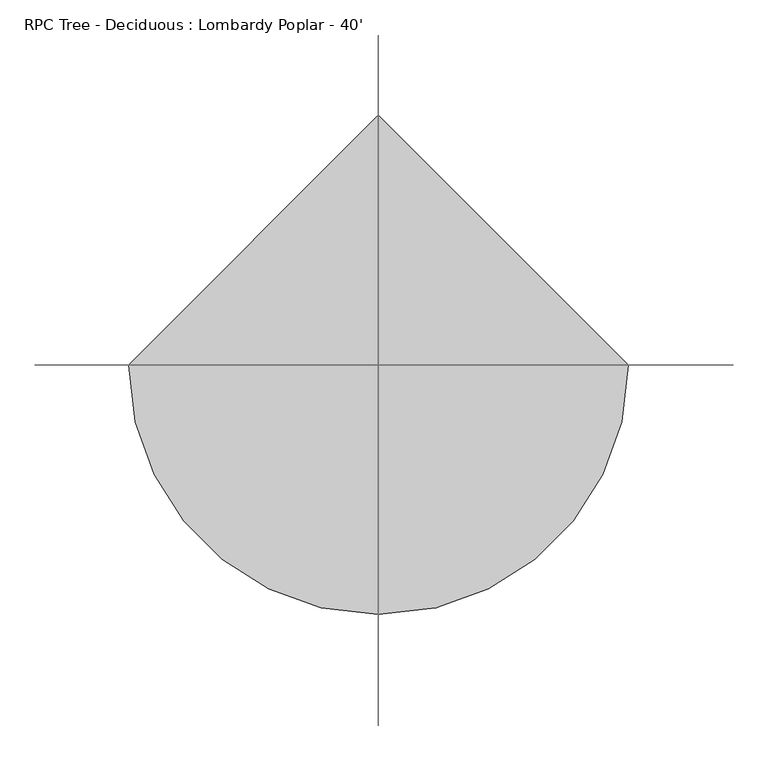
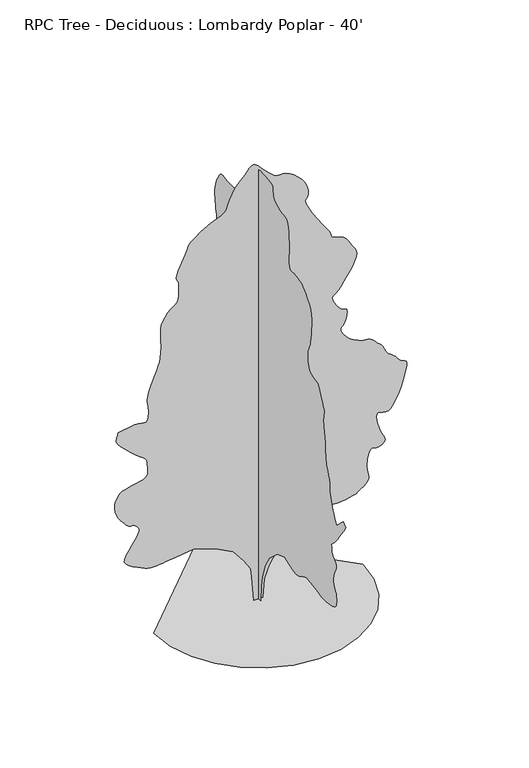
"""IFC4 building model written with IfcOpenShell, lengths in millimetres: geographic element geometry, RPC Tree - Deciduous : Lombardy Poplar - 40'."""

import ifcopenshell
import ifcopenshell.guid

model = None  # the IFC model being written
_history = None  # IfcOwnerHistory: only IFC2X3 demands one
_inside = {}  # id of a spatial element -> (the spatial element, [elements in it])
_under = {}  # id of a project, library or spatial element -> (it, [spatial elements below it])
_declared = {}  # id of a project -> (the project, [libraries it declares])
_typed = {}  # id of a type object -> (the type object, [elements of that type])
_made_of = {}  # id of a material, layer set ... -> (it, [elements and type objects made of it])


def new_model(schema):
    """Start an empty IFC model of exactly this schema.

    Asked for "IFC4X3", IfcOpenShell would pick the latest addendum, in which some entities
    have other attributes; the version numbers below select the first issue.
    IFC2X3 requires an IfcOwnerHistory on every rooted entity: one is made here for all.
    """
    global model, _history
    if schema == "IFC4X3":
        model = ifcopenshell.file(schema_version=(4, 3, 0, 0))
    else:
        model = ifcopenshell.file(schema=schema)
    _inside.clear()
    _under.clear()
    _declared.clear()
    _typed.clear()
    _made_of.clear()
    _history = None
    if model.schema == "IFC2X3":
        org = make("IfcOrganization", Name="unknown")
        user = make(
            "IfcPersonAndOrganization",
            ThePerson=make("IfcPerson", FamilyName="unknown"),
            TheOrganization=org,
        )
        app = make(
            "IfcApplication",
            ApplicationDeveloper=org,
            Version="unknown",
            ApplicationFullName="unknown",
            ApplicationIdentifier="unknown",
        )
        _history = make(
            "IfcOwnerHistory",
            OwningUser=user,
            OwningApplication=app,
            ChangeAction="ADDED",
            CreationDate=0,
        )
    return model


def make(cls, **values):
    """One entity of the class cls with the attributes given. An attribute that is None is left unset."""
    return model.create_entity(
        cls, **{name: value for name, value in values.items() if value is not None}
    )


def rooted(cls, **values):
    """An entity with a GlobalId (a new one), such as an element, a storey or a relation."""
    return make(cls, GlobalId=ifcopenshell.guid.new(), OwnerHistory=_history, **values)


def si_unit(unit_type, name, prefix=None):
    """IfcSIUnit, for example si_unit("LENGTHUNIT", "METRE", prefix="MILLI")."""
    return make("IfcSIUnit", UnitType=unit_type, Prefix=prefix, Name=name)


def assignment(units):
    """IfcUnitAssignment: the units of a project."""
    return None if units is None else make("IfcUnitAssignment", Units=units)


def point(xyz):
    """IfcCartesianPoint."""
    return None if xyz is None else make("IfcCartesianPoint", Coordinates=xyz)


def direction(xyz):
    """IfcDirection."""
    return None if xyz is None else make("IfcDirection", DirectionRatios=xyz)


def frame(location, z_axis=None, x_axis=None):
    """IfcAxis2Placement3D, a coordinate frame: its origin and axes. An axis left out is left unset."""
    return make(
        "IfcAxis2Placement3D",
        Location=point(location),
        Axis=direction(z_axis),
        RefDirection=direction(x_axis),
    )


def origin():
    """The frame at (0, 0, 0) with its axes left unset."""
    return frame((0.0, 0.0, 0.0))


def place(relative_to, where):
    """IfcLocalPlacement: puts the frame where relative to a parent placement (None: the world)."""
    return make(
        "IfcLocalPlacement", PlacementRelTo=relative_to, RelativePlacement=where
    )


def context(
    kind, dimensions, precision=None, world=None, true_north=None, identifier=None
):
    """IfcGeometricRepresentationContext, for example the 3D "Model" context."""
    return make(
        "IfcGeometricRepresentationContext",
        ContextIdentifier=identifier,
        ContextType=kind,
        CoordinateSpaceDimension=dimensions,
        Precision=precision,
        WorldCoordinateSystem=world,
        TrueNorth=true_north,
    )


def project(units=None, contexts=None):
    """IfcProject with its units and contexts."""
    return rooted(
        "IfcProject",
        Name="project",
        RepresentationContexts=contexts,
        UnitsInContext=assignment(units),
    )


def spatial(cls, under=None, at=None, **own):
    """A site, building, storey or space (cls), placed at a placement, below another one or the project."""
    s = rooted(cls, ObjectPlacement=at, **own)
    if under is not None:
        _under.setdefault(under.id(), (under, []))[1].append(s)
    return s


def point_list(points):
    """IfcCartesianPointList2D or 3D."""
    cls = (
        "IfcCartesianPointList2D" if len(points[0]) == 2 else "IfcCartesianPointList3D"
    )
    return make(cls, CoordList=points)


def triangles(points, corners, closed=None, point_numbers=None):
    """IfcTriangulatedFaceSet: each triangle names its three corners, points numbered from 1."""
    return make(
        "IfcTriangulatedFaceSet",
        Coordinates=point_list(points),
        Closed=closed,
        CoordIndex=corners,
        PnIndex=point_numbers,
    )


def shape(context_of_items, identifier, shape_type, items):
    """IfcShapeRepresentation: the items that make up one representation, for example the "Body"."""
    return make(
        "IfcShapeRepresentation",
        ContextOfItems=context_of_items,
        RepresentationIdentifier=identifier,
        RepresentationType=shape_type,
        Items=items,
    )


def source(mapping_origin, context_of_items, identifier, shape_type, items):
    """IfcRepresentationMap: a shape defined once, which mapped items show again and again."""
    return make(
        "IfcRepresentationMap",
        MappingOrigin=mapping_origin,
        MappedRepresentation=shape(context_of_items, identifier, shape_type, items),
    )


def transform(
    local_origin,
    x_axis=None,
    y_axis=None,
    z_axis=None,
    scale=None,
    scale2=None,
    scale3=None,
    uniform=True,
):
    """IfcCartesianTransformationOperator3D, or its non-uniform kind. x_axis, y_axis, z_axis: its Axis1, 2, 3."""
    if uniform:
        return make(
            "IfcCartesianTransformationOperator3D",
            Axis1=direction(x_axis),
            Axis2=direction(y_axis),
            LocalOrigin=point(local_origin),
            Scale=scale,
            Axis3=direction(z_axis),
        )
    return make(
        "IfcCartesianTransformationOperator3DnonUniform",
        Axis1=direction(x_axis),
        Axis2=direction(y_axis),
        LocalOrigin=point(local_origin),
        Scale=scale,
        Axis3=direction(z_axis),
        Scale2=scale2,
        Scale3=scale3,
    )


def mapped(mapping_source, mapping_target):
    """IfcMappedItem: shows the shape of a source again, moved by a transform."""
    return make(
        "IfcMappedItem", MappingSource=mapping_source, MappingTarget=mapping_target
    )


def made_of(thing, what):
    """Note that an element or type object is made of a material, layer set ...; save() writes the relation."""
    if what is not None:
        _made_of.setdefault(what.id(), (what, []))[1].append(thing)
    return thing


def element(
    cls,
    number,
    at=None,
    inside=None,
    cuts=None,
    type_object=None,
    material=None,
    context=None,
    identifier="Body",
    shape_type=None,
    held_by="IfcProductDefinitionShape",
    body=None,
    shapes=None,
    **own,
):
    """One element of the class cls, such as IfcWall. Its Tag is "e" and its number.

    at: its placement. inside: the storey or other place that contains it. cuts: it is an
    opening in that element (IfcRelVoidsElement). A single representation is given by context,
    identifier, shape_type and body (its items); several are given by shapes. held_by: the class
    of the entity that holds the representations. save() writes the other relations.
    """
    e = rooted(cls, Tag="e%d" % number, ObjectPlacement=at, **own)
    if body is not None:
        shapes = [shape(context, identifier, shape_type, body)]
    if shapes is not None:
        e.Representation = make(held_by, Representations=shapes)
    if inside is not None:
        _inside.setdefault(inside.id(), (inside, []))[1].append(e)
    if cuts is not None:
        rooted(
            "IfcRelVoidsElement", RelatingBuildingElement=cuts, RelatedOpeningElement=e
        )
    if type_object is not None:
        _typed.setdefault(type_object.id(), (type_object, []))[1].append(e)
    return made_of(e, material)


def aggregate(whole, parts):
    """IfcRelAggregates: a whole, such as a stair, and the parts it consists of."""
    return rooted("IfcRelAggregates", RelatingObject=whole, RelatedObjects=parts)


def save(model, path):
    """Write the relations noted so far, then the file.

    IfcRelAggregates (storeys below a building ...), IfcRelContainedInSpatialStructure (elements
    in a storey), IfcRelDefinesByType, IfcRelAssociatesMaterial and IfcRelDeclares: one each for
    every whole, place, type object, material and project.
    """
    for whole, parts in _under.values():
        aggregate(whole, parts)
    for where, things in _inside.values():
        rooted(
            "IfcRelContainedInSpatialStructure",
            RelatedElements=things,
            RelatingStructure=where,
        )
    for kind, things in _typed.values():
        rooted("IfcRelDefinesByType", RelatedObjects=things, RelatingType=kind)
    for what, things in _made_of.values():
        rooted("IfcRelAssociatesMaterial", RelatedObjects=things, RelatingMaterial=what)
    for by, libraries in _declared.values():
        rooted("IfcRelDeclares", RelatingContext=by, RelatedDefinitions=libraries)
    model.write(path)


def rpc_tree_deciduous_lombardy_poplar_40_01077960(model_context):
    return source(origin(), model_context, "Body", "Tessellation", [
        triangles([(0.0009695, 113.8156909, 0.0), (0.0009695, -104.8345258, 0.0), (0.0009695, -123.055434, 437.3009239), (0.0009695, -177.7179314, 728.8340738), (0.0009695, -323.483707, 1129.6911467), (0.0009695, -505.6928613, 1439.4461494), (0.0009695, -870.1086628, 1767.420607), (0.0009695, -1216.3049732, 1894.9664555), (0.0009695, -1398.5142002, 1822.0838402), (0.0009695, -1476.390406, 1795.1523445), (0.0009695, -1552.9941605, 1770.6083485), (0.0009695, -1627.0451637, 1750.8472), (0.0009695, -1697.2735806, 1738.2588696), (0.0009695, -1762.3991112, 1735.2286766), (0.0009695, -1821.1516296, 1744.1542946), (0.0009695, -1872.2563591, 1767.420607), (0.0009695, -1919.1091679, 1797.0624023), (0.0009695, -1965.9644474, 1823.8364948), (0.0009695, -2012.8172562, 1848.2204716), (0.0009695, -2059.6700649, 1870.6891582), (0.0009695, -2106.5227283, 1891.7279903), (0.0009695, -2153.3780079, 1911.8067066), (0.0009695, -2200.2308167, 1931.4103065), (0.0009695, -2582.8711235, 1876.7470734), (0.0009695, -2649.2156204, 1861.2353748), (0.0009695, -2715.4080917, 1846.3611374), (0.0009695, -2781.27006, 1832.7619675), (0.0009695, -2846.6750793, 1821.0754715), (0.0009695, -2911.4196739, 1811.9366398), (0.0009695, -2975.3765259, 1805.987875), (0.0009695, -3038.3939003, 1803.8619873), (0.0009695, -3111.6472778, 1806.252103), (0.0009695, -3200.5217949, 1814.0625275), (0.0009695, -3296.0764275, 1828.2459641), (0.0009695, -3389.4213112, 1849.7596218), (0.0009695, -3471.5901329, 1879.5614365), (0.0009695, -3533.6930283, 1918.6062916), (0.0009695, -3566.7892639, 1967.8516869), (0.0009695, -3579.2353065, 2021.4507408), (0.0009695, -3585.9154221, 2073.1371208), (0.0009695, -3587.8205383, 2123.2333363), (0.0009695, -3585.9154221, 2172.0521587), (0.0009695, -3581.1401321, 2219.915807), (0.0009695, -3574.4347275, 2267.139378), (0.0009695, -3566.7892639, 2314.0455265), (0.0009695, -3532.0422569, 2353.5170998), (0.0009695, -3499.7078934, 2395.5361919), (0.0009695, -3472.1235306, 2442.6555542), (0.0009695, -3451.7273918, 2497.4231415), (0.0009695, -3440.907122, 2562.3988266), (0.0009695, -3441.9992065, 2640.0972816), (0.0009695, -3457.4677391, 2733.1372421), (0.0009695, -3484.5187042, 2825.1865654), (0.0009695, -3515.3799019, 2900.6752716), (0.0009695, -3544.9708282, 2963.0830902), (0.0009695, -3568.1862717, 3015.940329), (0.0009695, -3579.9210205, 3062.7525879), (0.0009695, -3575.0695724, 3106.9993057), (0.0009695, -3548.5775848, 3152.2110809), (0.0009695, -3509.7918709, 3193.1050964), (0.0009695, -3472.6063499, 3225.0836678), (0.0009695, -3438.6212151, 3252.6171616), (0.0009695, -3409.3857903, 3280.1253662), (0.0009695, -3386.5511375, 3312.1039375), (0.0009695, -3371.6668716, 3352.997953), (0.0009695, -3366.3581841, 3407.3030685), (0.0009695, -3362.7005585, 3460.5158089), (0.0009695, -3354.9027786, 3498.4634926), (0.0009695, -3347.7145546, 3525.8699593), (0.0009695, -3345.9620453, 3547.5360786), (0.0009695, -3354.4202499, 3568.2624298), (0.0009695, -3377.8388786, 3592.7987228), (0.0009695, -3421.0188011, 3625.9458275), (0.0009695, -3481.5215034, 3679.8698616), (0.0009695, -3552.5654228, 3760.5655174), (0.0009695, -3632.3465996, 3863.5624283), (0.0009695, -3719.1381042, 3984.4155167), (0.0009695, -3811.2130074, 4118.6541252), (0.0009695, -3906.7676399, 4261.8084686), (0.0009695, -4004.1003616, 4409.432888), (0.0009695, -3894.7788368, 4518.779702), (0.0009695, -3749.0086647, 4391.221209), (0.0009695, -3603.2382019, 4227.2390671), (0.0009695, -3579.7434151, 4258.785688), (0.0009695, -3555.9689941, 4292.2630051), (0.0009695, -3531.5088593, 4329.5499733), (0.0009695, -3506.1342453, 4372.5775795), (0.0009695, -3479.4643616, 4423.2506493), (0.0009695, -3451.1939941, 4483.4992973), (0.0009695, -3421.0188011, 4555.2033508), (0.0009695, -3390.0055779, 4628.5837555), (0.0009695, -3360.2623352, 4695.8683113), (0.0009695, -3333.0587631, 4762.2383881), (0.0009695, -3309.6910034, 4832.7233299), (0.0009695, -3291.4028755, 4912.4536377), (0.0009695, -3279.5158104, 5006.5351044), (0.0009695, -3275.248629, 5120.0473618), (0.0009695, -3267.0697678, 5234.8554703), (0.0009695, -3245.5050957, 5333.3820145), (0.0009695, -3215.0252701, 5421.7481323), (0.0009695, -3180.0747871, 5505.9238083), (0.0009695, -3145.0993057, 5592.0551788), (0.0009695, -3114.6191895, 5686.1110657), (0.0009695, -3093.0545174, 5794.238768), (0.0009695, -3079.5672592, 5892.1298859), (0.0009695, -3069.8899429, 5959.4403122), (0.0009695, -3063.4130127, 6007.9286316), (0.0009695, -3059.4760437, 6049.4319122), (0.0009695, -3057.4691895, 6095.6854843), (0.0009695, -3056.7073174, 6158.5246719), (0.0009695, -3056.6055794, 6249.735965), (0.0009695, -3052.5671631, 6343.1320084), (0.0009695, -3042.1532639, 6412.2958099), (0.0009695, -3027.9291321, 6468.709227), (0.0009695, -3012.4097305, 6523.8523727), (0.0009695, -2998.1858894, 6589.2065231), (0.0009695, -2987.7716995, 6676.2017944), (0.0009695, -2983.7332832, 6796.3688782), (0.0009695, -2989.2957344, 6908.7381821), (0.0009695, -3001.5638809, 6976.78461), (0.0009695, -3013.8576073, 7018.6948425), (0.0009695, -3019.4200584, 7052.6288177), (0.0009695, -3011.6222786, 7096.7737976), (0.0009695, -2983.7332832, 7169.2908829), (0.0009695, -2929.0723755, 7288.340593), (0.0009695, -2866.7410057, 7418.1088348), (0.0009695, -2818.7857933, 7514.4256302), (0.0009695, -2782.7688057, 7582.8528488), (0.0009695, -2756.3021072, 7628.9541046), (0.0009695, -2737.0233421, 7658.3418457), (0.0009695, -2722.5201576, 7676.5535248), (0.0009695, -2710.4043274, 7689.2027527), (0.0009695, -2636.5666832, 7701.2421341), (0.0009695, -2564.8117607, 7715.3901077), (0.0009695, -2497.1818771, 7733.6523651), (0.0009695, -2435.7748695, 7758.1380798), (0.0009695, -2382.6507866, 7790.9296829), (0.0009695, -2339.8900246, 7834.0584457), (0.0009695, -2309.5548122, 7889.6335419), (0.0009695, -2289.3160767, 7951.0257248), (0.0009695, -2274.8152176, 8010.5377899), (0.0009695, -2265.0921192, 8068.4243729), (0.0009695, -2259.1968395, 8125.0662643), (0.0009695, -2256.1691174, 8180.7425171), (0.0009695, -2255.0515984, 8235.7589264), (0.0009695, -2254.8940498, 8290.4707031), (0.0009695, -2285.970932, 8345.7405853), (0.0009695, -2316.0901691, 8404.491069), (0.0009695, -2344.2968777, 8470.25159), (0.0009695, -2369.6358833, 8546.5277481), (0.0009695, -2391.1521572, 8636.8495605), (0.0009695, -2407.8857288, 8744.6726303), (0.0009695, -2418.8812786, 8873.551973), (0.0009695, -2430.0903328, 9004.9206985), (0.0009695, -2443.8493767, 9121.3031296), (0.0009695, -2453.7833633, 9227.8303482), (0.0009695, -2453.5168098, 9329.5572784), (0.0009695, -2436.6765587, 9431.5888412), (0.0009695, -2396.8874176, 9539.0561188), (0.0009695, -2327.7766651, 9657.0390335), (0.0009695, -2247.8811058, 9768.2398041), (0.0009695, -2177.228587, 9854.8798645), (0.0009695, -2111.6764835, 9921.4269653), (0.0009695, -2047.0792637, 9972.3796692), (0.0009695, -1979.2969185, 10012.156311), (0.0009695, -1904.1815907, 10045.2519653), (0.0009695, -1817.5931259, 10076.1128723), (0.0009695, -1725.5334835, 10094.8326599), (0.0009695, -1638.891679, 10096.3058258), (0.0009695, -1560.8554539, 10092.3688568), (0.0009695, -1494.6124043, 10094.8326599), (0.0009695, -1443.3501263, 10115.4325653), (0.0009695, -1410.2540359, 10166.0038971), (0.0009695, -1398.5142002, 10258.3319824), (0.0009695, -1400.4267288, 10362.6756134), (0.0009695, -1404.8895378, 10448.1971375), (0.0009695, -1409.9898079, 10525.1087219), (0.0009695, -1413.8125397, 10603.619046), (0.0009695, -1414.4501461, 10693.9414398), (0.0009695, -1409.9898079, 10806.2345856), (0.0009695, -1398.5142002, 10950.7350677), (0.0009695, -1382.6849339, 11097.4458801), (0.0009695, -1365.5779839, 11211.9737732), (0.0009695, -1345.9235149, 11297.8255096), (0.0009695, -1322.4438435, 11358.4811096), (0.0009695, -1293.8637566, 11397.4694275), (0.0009695, -1258.9083321, 11418.297226), (0.0009695, -1216.3049732, 11424.470105), (0.0009695, -1155.4822323, 11429.9813965), (0.0009695, -1073.3006933, 11446.3641174), (0.0009695, -979.6484882, 11473.2380585), (0.0009695, -884.3986336, 11510.3218414), (0.0009695, -797.4393339, 11557.2608368), (0.0009695, -728.6460766, 11613.8015717), (0.0009695, -687.9020519, 11679.5615112), (0.0009695, -672.8677952, 11749.3607391), (0.0009695, -668.0341513, 11816.289212), (0.0009695, -663.5180752, 11877.4785004), (0.0009695, -649.4413908, 11930.0811035), (0.0009695, -615.9210531, 11971.2041748), (0.0009695, -553.0790314, 11997.9757965), (0.0009695, -451.0296281, 12007.5263763), (0.0009695, -327.7864603, 12011.2087097), (0.0009695, -210.2816959, 12019.0070709), (0.0009695, -102.0189364, 12026.1694244), (0.0009695, -6.5056406, 12027.9216431), (0.0009695, 72.7523407, 12019.4895996), (0.0009695, 132.2489498, 11996.0700989), (0.0009695, 168.4781792, 11952.8657593), (0.0009695, 190.2581361, 11903.7920105), (0.0009695, 211.0820467, 11861.400412), (0.0009695, 234.4553475, 11819.0076508), (0.0009695, 263.8852554, 11769.9094849), (0.0009695, 302.8767344, 11707.4505066), (0.0009695, 354.9364746, 11624.9008942), (0.0009695, 423.5697126, 11515.57966), (0.0009695, 499.5867296, 11399.1204895), (0.0009695, 572.09851, 11297.9778259), (0.0009695, 642.0601553, 11209.5867096), (0.0009695, 710.4292379, 11131.3798553), (0.0009695, 778.1582434, 11060.8446259), (0.0009695, 846.2072874, 10995.3881561), (0.0009695, 915.531399, 10932.4978088), (0.0009695, 983.7404623, 10880.5556305), (0.0009695, 1048.444289, 10847.0786041), (0.0009695, 1110.5954372, 10828.282077), (0.0009695, 1171.1565662, 10820.3069824), (0.0009695, 1231.077618, 10819.3407623), (0.0009695, 1291.3160923, 10821.5766724), (0.0009695, 1352.8322502, 10823.1765747), (0.0009695, 1419.1287849, 10828.7646057), (0.0009695, 1490.5254444, 10841.0324615), (0.0009695, 1563.194846, 10853.3014801), (0.0009695, 1633.3164379, 10858.8639313), (0.0009695, 1697.0626923, 10851.0655701), (0.0009695, 1750.6084064, 10823.1765747), (0.0009695, 1790.1333195, 10768.5159576), (0.0009695, 1824.1844387, 10700.9526398), (0.0009695, 1861.7408672, 10636.2333344), (0.0009695, 1899.617189, 10570.5745514), (0.0009695, 1934.6234825, 10500.1404785), (0.0009695, 1963.5743317, 10421.0953033), (0.0009695, 1983.2847565, 10329.6299561), (0.0009695, 1990.5617832, 10221.8830444), (0.0009695, 1988.4357502, 10111.0130676), (0.0009695, 1982.4871307, 10010.9877777), (0.0009695, 1973.3507698, 9919.2433777), (0.0009695, 1961.6642738, 9833.2381622), (0.0009695, 1948.0651039, 9750.4350769), (0.0009695, 1933.1908665, 9668.2656738), (0.0009695, 1917.6791679, 9584.1667374), (0.0009695, 1914.3314072, 9505.3761978), (0.0009695, 1931.0649788, 9438.0663528), (0.0009695, 1961.1842159, 9378.0967575), (0.0009695, 1997.9989746, 9321.3025497), (0.0009695, 2034.813588, 9263.5682831), (0.0009695, 2064.9328251, 9200.7290955), (0.0009695, 2081.6663967, 9128.6439606), (0.0009695, 2081.1888096, 9058.6668365), (0.0009695, 2066.6854797, 9001.7964706), (0.0009695, 2041.9840805, 8953.1808334), (0.0009695, 2010.9071983, 8908.0707962), (0.0009695, 1977.2826519, 8861.6904877), (0.0009695, 1944.9307022, 8809.2646179), (0.0009695, 1917.6791679, 8745.9934799), (0.0009695, 1901.8472855, 8673.7048691), (0.0009695, 1900.361475, 8598.2164536), (0.0009695, 1911.9412914, 8520.8229218), (0.0009695, 1935.3142834, 8442.7939636), (0.0009695, 1969.2055286, 8365.374852), (0.0009695, 2012.3422852, 8289.8864365), (0.0009695, 2063.4443985, 8217.5978256), (0.0009695, 2116.1951031, 8158.060762), (0.0009695, 2166.3955273, 8113.7884644), (0.0009695, 2215.9584904, 8075.6123062), (0.0009695, 2266.796521, 8034.2101822), (0.0009695, 2320.8222931, 7980.4134659), (0.0009695, 2379.9457191, 7904.924469), (0.0009695, 2446.0820892, 7798.5239868), (0.0009695, 2515.4595406, 7684.1478287), (0.0009695, 2583.8870499, 7588.5931961), (0.0009695, 2652.6194824, 7508.3039108), (0.0009695, 2722.9518173, 7439.8511124), (0.0009695, 2796.1546165, 7379.653624), (0.0009695, 2873.4972794, 7324.2558426), (0.0009695, 2956.2759476, 7270.103334), (0.0009695, 3039.9940933, 7227.3042023), (0.0009695, 3119.5720848, 7202.0063278), (0.0009695, 3195.3148453, 7185.0137604), (0.0009695, 3267.5522964, 7167.0555542), (0.0009695, 3336.6149414, 7138.9125046), (0.0009695, 3402.807122, 7091.3130844), (0.0009695, 3466.4593414, 7015.0113464), (0.0009695, 3525.2604034, 6921.5903046), (0.0009695, 3575.4506538, 6829.7441666), (0.0009695, 3615.1508469, 6741.0728348), (0.0009695, 3642.3797081, 6657.2023727), (0.0009695, 3655.3082794, 6579.6815231), (0.0009695, 3651.9552864, 6510.1619293), (0.0009695, 3630.4414833, 6450.1673355), (0.0009695, 3590.004998, 6392.5348068), (0.0009695, 3534.6075073, 6330.4316208), (0.0009695, 3469.3295151, 6266.1192673), (0.0009695, 3399.2512344, 6201.7813339), (0.0009695, 3329.5028755, 6139.6781479), (0.0009695, 3265.1646515, 6082.0456192), (0.0009695, 3211.3676445, 6031.0934967), (0.0009695, 3161.7869499, 5985.0939789), (0.0009695, 3109.3613708, 5939.7298874), (0.0009695, 3057.8758507, 5893.4001572), (0.0009695, 3011.1906189, 5844.5304657), (0.0009695, 2973.1159081, 5791.5209106), (0.0009695, 2947.4366615, 5732.7710083), (0.0009695, 2938.0386887, 5666.680275), (0.0009695, 2934.1778778, 5597.4141541), (0.0009695, 2924.8816429, 5529.7235184), (0.0009695, 2913.6547119, 5463.0235199), (0.0009695, 2904.0535538, 5396.6025742), (0.0009695, 2899.5323181, 5329.8764145), (0.0009695, 2903.6218941, 5262.2113586), (0.0009695, 2919.8270096, 5192.9452377), (0.0009695, 2944.8458313, 5126.3719757), (0.0009695, 2972.7351173, 5066.5046997), (0.0009695, 3003.0117577, 5012.2248734), (0.0009695, 3035.1935143, 4962.3901245), (0.0009695, 3068.8231476, 4915.908078), (0.0009695, 3103.4178383, 4871.6613602), (0.0009695, 3138.4697685, 4828.5323067), (0.0009695, 3181.1415825, 4835.3141602), (0.0009695, 3222.035598, 4836.0760323), (0.0009695, 3259.4243042, 4824.696785), (0.0009695, 3291.5807716, 4795.1567276), (0.0009695, 3316.7013313, 4741.4102989), (0.0009695, 3333.0587631, 4657.3619408), (0.0009695, 3338.9008484, 4536.9916718), (0.0009695, 3338.9008484, 3935.6984322), (0.0009695, 3345.6065437, 3757.6444748), (0.0009695, 3361.2273926, 3611.1377197), (0.0009695, 3379.0582809, 3492.0371407), (0.0009695, 3392.4440918, 3396.2031647), (0.0009695, 3394.6791298, 3319.4953468), (0.0009695, 3379.0582809, 3257.747953), (0.0009695, 3338.9008484, 3206.8719887), (0.0009695, 3281.573243, 3178.2461197), (0.0009695, 3221.7053856, 3174.1568344), (0.0009695, 3163.4380119, 3176.747374), (0.0009695, 3110.9106949, 3168.187722), (0.0009695, 3068.2388809, 3130.6466995), (0.0009695, 3039.6130119, 3046.21726), (0.0009695, 3029.1482437, 2897.119384), (0.0009695, 3036.0571243, 2732.8070297), (0.0009695, 3053.1514297, 2608.9823204), (0.0009695, 3075.0460236, 2517.0268867), (0.0009695, 3096.3057724, 2448.3400909), (0.0009695, 3111.4949615, 2394.3144642), (0.0009695, 3115.2034561, 2346.3441364), (0.0009695, 3102.0208305, 2295.8261444), (0.0009695, 3089.0669701, 2254.1778145), (0.0009695, 3089.803553, 2232.6106716), (0.0009695, 3093.4355988, 2222.1992432), (0.0009695, 3089.0669701, 2214.0179111), (0.0009695, 3065.9021049, 2199.1436737), (0.0009695, 3013.0954445, 2168.6510582), (0.0009695, 2919.8270096, 2113.6169174), (0.0009695, 2822.3419716, 2052.8450455), (0.0009695, 2753.55867, 2008.9666191), (0.0009695, 2697.5010452, 1978.7940422), (0.0009695, 2638.2683235, 1959.1395733), (0.0009695, 2559.9350235, 1946.8154709), (0.0009695, 2446.5088074, 1938.6341389), (0.0009695, 2282.0948605, 1931.4103065), (0.0009695, 2105.8903542, 1933.6938881), (0.0009695, 1963.4702682, 1951.9132702), (0.0009695, 1848.4591198, 1979.6982021), (0.0009695, 1754.4869488, 2010.665934), (0.0009695, 1675.1755108, 2038.4483952), (0.0009695, 1604.1522297, 2056.670248), (0.0009695, 1535.0414772, 2058.9536842), (0.0009695, 1460.510416, 2049.0198429), (0.0009695, 1378.3312752, 2035.2631245), (0.0009695, 1289.7769421, 2018.3163391), (0.0009695, 1196.1221935, 1998.8218895), (0.0009695, 1098.6447859, 1977.4122952), (0.0009695, 998.6146271, 1954.7301041), (0.0009695, 897.3120169, 1931.4103065), (0.0009695, 532.8936719, 1639.8747585), (0.0009695, 314.2457534, 1166.1349977), (0.0009695, 168.4781792, 601.2881527), (120.1776209, 0.0005334, 0.0085345), (-116.69275, 0.0005334, 0.0085345), (-171.3552383, 0.0004849, 655.9590162), (-207.7973272, 0.0004849, 911.0508585), (-390.006209, 0.0004607, 1202.5839357), (-663.3174334, 0.0004364, 1548.7803188), (-1137.0596649, 0.0004122, 1803.8721611), (-1720.1284355, 0.0004122, 1986.078772), (-2193.8681236, 0.0004122, 1931.4180096), (-2467.1819641, 0.0004122, 1894.9766293), (-2533.7959213, 0.0004122, 1885.46689), (-2607.4327057, 0.0004122, 1874.6820831), (-2686.1473778, 0.0004122, 1865.812421), (-2768.0621452, 0.0004122, 1862.0405582), (-2851.2468933, 0.0004122, 1866.556707), (-2933.7967964, 0.0004122, 1882.5459927), (-3013.8067383, 0.0004122, 1913.1960114), (-3104.2814484, 0.0004122, 1955.5886272), (-3210.9865631, 0.0004122, 2004.6715324), (-3321.222567, 0.0004122, 2060.4522846), (-3422.2126236, 0.0004122, 2122.9234715), (-3501.2066391, 0.0003879, 2192.0875637), (-3545.4533569, 0.0003879, 2267.9445614), (-3542.2021019, 0.0003879, 2350.4969353), (-3495.1869484, 0.0003879, 2447.2326004), (-3424.930481, 0.0003879, 2559.9094437), (-3343.8031654, 0.0003637, 2679.898922), (-3264.2757523, 0.0003637, 2798.6437088), (-3198.7692856, 0.0003637, 2907.4824142), (-3159.7295174, 0.0003394, 2997.8300972), (-3159.5772011, 0.0003394, 3061.1015259), (-3182.9958298, 0.0003394, 3103.1893639), (-3206.4147491, 0.0003394, 3136.6411011), (-3229.8589577, 0.0003394, 3162.9554832), (-3253.2775864, 0.0003394, 3183.5039383), (-3276.6962151, 0.0003394, 3199.7599228), (-3300.1404236, 0.0003394, 3213.1457336), (-3323.559343, 0.0003394, 3225.1089569), (-3347.1558678, 0.0003394, 3221.5783585), (-3371.6921608, 0.0003394, 3220.486274), (-3398.1335701, 0.0003394, 3224.1438995), (-3427.4704422, 0.0003394, 3234.9897491), (-3460.6175468, 0.0003394, 3255.3858879), (-3498.5396507, 0.0003394, 3287.7199608), (-3542.2021019, 0.0003394, 3334.4304817), (-3593.6370438, 0.0003394, 3395.5174507), (-3650.1519081, 0.0003152, 3468.3897469), (-3705.7270042, 0.0003152, 3551.4730476), (-3754.2664833, 0.0003152, 3643.1668694), (-3789.7500732, 0.0003152, 3741.8713097), (-3806.1330849, 0.0002909, 3845.9855942), (-3797.2937988, 0.0002909, 3953.9354004), (-3771.4366562, 0.0002909, 4051.5730453), (-3739.8138771, 0.0002909, 4128.1791252), (-3701.2057686, 0.0002909, 4187.2342415), (-3654.2920624, 0.0002667, 4232.2937004), (-3597.828067, 0.0002667, 4266.812233), (-3530.518222, 0.0002667, 4294.3457268), (-3451.117836, 0.0002667, 4318.3486221), (-3356.8078949, 0.0002667, 4338.3131012), (-3252.3378181, 0.0002667, 4355.4326958), (-3147.5122398, 0.0002667, 4375.7270966), (-3052.2622398, 0.0002667, 4405.2674446), (-2976.4689011, 0.0002667, 4450.0981384), (-2929.9868546, 0.0002667, 4516.2906097), (-2922.6971832, 0.0002667, 4609.8895477), (-2933.5936111, 0.0002425, 4707.6283493), (-2938.4197701, 0.0002425, 4784.9713028), (-2942.3058701, 0.0002425, 4846.0582718), (-2950.332415, 0.0002425, 4895.0291199), (-2967.578746, 0.0002425, 4936.0504532), (-2999.2018158, 0.0002425, 4973.2359741), (-3050.2556763, 0.0002425, 5010.7517075), (-3135.4978569, 0.0002182, 5072.041571), (-3254.8777794, 0.0002182, 5168.7141586), (-3391.1232422, 0.0002182, 5287.0778641), (-3527.0637817, 0.0002182, 5413.3916656), (-3645.4783562, 0.000194, 5533.9906998), (-3729.1459236, 0.000194, 5635.1333633), (-3760.8704407, 0.000194, 5703.129213), (-3759.2702477, 0.000194, 5747.3247711), (-3754.799881, 0.000194, 5786.7456207), (-3747.9418694, 0.000194, 5822.178923), (-3739.1787415, 0.0001697, 5854.4112579), (-3728.9933167, 0.0001697, 5884.2815277), (-3717.8428345, 0.0001697, 5912.5263153), (-3706.2095329, 0.0001697, 5940.0089401), (-3268.8984352, 0.0001697, 6012.8818176), (-3174.1312546, 0.0001697, 6014.48172), (-3093.0545174, 0.0001697, 5998.8605804), (-3026.0240158, 0.0001697, 5982.2743835), (-2973.319384, 0.0001697, 5981.0046936), (-2935.2955421, 0.0001697, 6011.2813339), (-2912.232415, 0.0001697, 6089.3864502), (-2904.4852135, 0.0001697, 6231.5242859), (-2910.9624344, 0.0001455, 6377.1421417), (-2925.0848282, 0.0001455, 6470.4870255), (-2938.9022987, 0.0001455, 6535.1301727), (-2944.4394608, 0.0001455, 6594.6678177), (-2933.6953491, 0.0001212, 6672.7217743), (-2898.7448662, 0.0001212, 6792.8126999), (-2831.5873375, 0.0001212, 6978.5879883), (-2754.346122, 9.7e-05, 7175.5649185), (-2693.3861801, 9.7e-05, 7325.0435852), (-2647.0567406, 9.7e-05, 7444.2456116), (-2613.8081886, 7.27e-05, 7550.3920395), (-2592.0150421, 7.27e-05, 7660.678331), (-2580.127977, 7.27e-05, 7792.3011108), (-2576.4956406, 4.85e-05, 7962.5064194), (-2580.0009499, 4.85e-05, 8135.9626923), (-2586.7063545, 4.85e-05, 8272.4363388), (-2590.8467995, 2.42e-05, 8381.8087326), (-2586.7063545, 2.42e-05, 8473.985083), (-2568.5455444, 2.42e-05, 8558.8211838), (-2530.6106506, 2.42e-05, 8646.1972458), (-2467.1819641, 0.0, 8746.0190598), (-2393.5550629, 0.0, 8838.8046753), (-2328.8511635, 0.0, 8903.8797729), (-2273.0728821, 0.0, 8949.1932861), (-2226.2200733, 0.0, 8982.7208908), (-2188.2902664, 0.0, 9012.4138458), (-2159.2860775, 0.0, 9046.2460831), (-2139.2048904, 0.0, 9092.1950226), (-2125.7124001, -2.42e-05, 9135.3493652), (-2116.0452576, -2.42e-05, 9162.8575699), (-2109.5630951, -2.42e-05, 9185.920697), (-2105.6338291, -2.42e-05, 9215.6642303), (-2103.6144756, -2.42e-05, 9263.2636505), (-2102.8701897, -2.42e-05, 9339.8700211), (-2102.7661263, -2.42e-05, 9456.6332428), (-2113.0708752, -4.85e-05, 9567.5549606), (-2136.1264446, -4.85e-05, 9634.4840149), (-2160.137043, -4.85e-05, 9680.3817947), (-2173.3094948, -4.85e-05, 9728.1846909), (-2163.855566, -4.85e-05, 9800.8540924), (-2119.9745235, -7.27e-05, 9921.3258087), (-2029.8808949, -7.27e-05, 10112.5618103), (-1939.4672276, -7.27e-05, 10305.830246), (-1888.8958958, -9.7e-05, 10431.5097839), (-1857.7656738, -9.7e-05, 10511.3165405), (-1825.6805683, -9.7e-05, 10566.8654755), (-1772.2389175, -9.7e-05, 10619.9006104), (-1677.0450188, -9.7e-05, 10692.0369049), (-1519.6973557, -0.0001212, 10804.9648956), (-1341.6868549, -0.0001212, 10917.309201), (-1195.5481733, -0.0001212, 10985.3806274), (-1077.4586517, -0.0001212, 11027.29086), (-983.5905441, -0.0001212, 11061.2248352), (-910.1237349, -0.0001212, 11105.3698151), (-853.2303326, -0.0001455, 11177.8874817), (-809.0852074, -0.0001455, 11296.9371918), (-759.9464916, -0.0001455, 11440.4714539), (-694.8717573, -0.0001697, 11572.8563965), (-620.2365601, -0.0001697, 11691.8293671), (-542.413585, -0.0001697, 11795.2079407), (-467.775808, -0.0001697, 11880.7294647), (-402.7036534, -0.0001697, 11946.1847717), (-353.5649014, -0.000194, 11989.3146973), (-315.2642959, -0.000194, 12029.8529205), (-276.9611651, -0.000194, 12081.541626), (-236.4299363, -0.000194, 12133.2303314), (-191.4351718, -0.000194, 12173.7685547), (-139.7475292, -0.000194, 12191.9802338), (-79.1353495, -0.000194, 12176.7404663), (-7.3676139, -0.000194, 12116.8731903), (68.4904824, -0.000194, 12035.3130524), (139.8862108, -0.000194, 11962.0605469), (206.8199341, -0.0001697, 11896.4517609), (269.290376, -0.0001697, 11837.8797546), (327.3013518, -0.0001697, 11785.6573608), (380.8469934, -0.0001697, 11739.1753143), (429.9324057, -0.0001697, 11697.7987701), (477.3160323, -0.0001697, 11672.4491547), (527.8899076, -0.0001697, 11666.8622864), (584.8366133, -0.0001697, 11669.5795624), (651.343891, -0.0001697, 11669.0970337), (730.6019165, -0.0001697, 11653.9584229), (825.7958879, -0.0001697, 11612.684198), (940.1160175, -0.0001455, 11533.7913391), (1053.1051964, -0.0001455, 11434.3508972), (1143.4680674, -0.0001455, 11338.4148926), (1213.1096741, -0.0001455, 11245.0194305), (1263.9477047, -0.0001455, 11153.2238708), (1297.8921444, -0.0001212, 11062.0631561), (1316.8558125, -0.0001212, 10970.5978088), (1322.7537083, -0.0001212, 10877.8371918), (1310.6404942, -0.0001212, 10807.3019623), (1283.8688725, -0.0001212, 10768.6426941), (1256.7747414, -0.0001212, 10740.1444336), (1243.7064983, -9.7e-05, 10700.2154755), (1259.0074539, -9.7e-05, 10627.1141235), (1317.0158318, -9.7e-05, 10499.1998383), (1432.0777039, -7.27e-05, 10294.7809204), (1568.3356659, -7.27e-05, 10074.4362305), (1681.0074223, -4.85e-05, 9906.365094), (1771.0503273, -4.85e-05, 9780.3565063), (1839.4167938, -4.85e-05, 9686.22388), (1887.067083, -4.85e-05, 9613.757373), (1914.9562237, -4.85e-05, 9552.772142), (1924.041861, -2.42e-05, 9493.0571823), (1943.5896503, -2.42e-05, 9444.2892288), (1995.6494087, -2.42e-05, 9415.2822784), (2070.3380184, -2.42e-05, 9394.5812164), (2157.7773033, -2.42e-05, 9370.6797684), (2248.0842911, -2.42e-05, 9332.0972397), (2331.3809509, -2.42e-05, 9267.4035141), (2397.7841652, -2.42e-05, 9165.0928986), (2454.6240097, 0.0, 9055.2379761), (2511.1467224, 0.0, 8968.9542892), (2560.341394, 0.0, 8896.3866257), (2595.190139, 0.0, 8827.6541931), (2608.6773972, 0.0, 8752.8512009), (2593.7931313, 2.42e-05, 8662.1230179), (2543.5520119, 2.42e-05, 8545.5876892), (2481.3447624, 2.42e-05, 8432.1260101), (2431.8886242, 2.42e-05, 8349.5508179), (2390.080275, 2.42e-05, 8286.457576), (2350.8220608, 4.85e-05, 8231.3138489), (2309.0163277, 4.85e-05, 8172.6656845), (2259.5600441, 4.85e-05, 8099.0312256), (2197.3530853, 4.85e-05, 7998.9553574), (2127.0206051, 4.85e-05, 7904.0355698), (2060.8307499, 7.27e-05, 7844.1677124), (2005.159148, 7.27e-05, 7805.3311295), (1966.378521, 7.27e-05, 7773.5051651), (1950.8666771, 7.27e-05, 7734.6685822), (1964.9992447, 7.27e-05, 7674.8007248), (2015.1464745, 7.27e-05, 7579.8815186), (2080.6452381, 7.27e-05, 7478.1545883), (2137.5387131, 9.7e-05, 7404.1387573), (2187.2590794, 9.7e-05, 7353.262793), (2231.2468014, 9.7e-05, 7320.852562), (2270.9265015, 9.7e-05, 7302.3106705), (2307.7412601, 9.7e-05, 7293.0141449), (2343.1207867, 9.7e-05, 7288.340593), (2346.839455, 9.7e-05, 7260.6544922), (2349.4429298, 9.7e-05, 7230.9109589), (2349.8136921, 9.7e-05, 7197.027562), (2346.839455, 9.7e-05, 7156.9212891), (2339.4022636, 9.7e-05, 7108.5341263), (2326.3873604, 0.0001212, 7049.7842239), (2306.6795517, 0.0001212, 6978.5879883), (2277.832766, 0.0001212, 6914.427951), (2243.2507198, 0.0001212, 6871.273027), (2210.5813477, 0.0001212, 6838.9901138), (2187.4724384, 0.0001212, 6807.3158844), (2181.5771587, 0.0001212, 6766.0922379), (2200.5406815, 0.0001212, 6705.1064255), (2252.0163185, 0.0001455, 6614.1747665), (2322.1379105, 0.0001455, 6519.5090332), (2391.3020027, 0.0001455, 6450.3452316), (2458.553421, 0.0001455, 6400.9424332), (2522.9372818, 0.0001455, 6365.5602905), (2583.5059685, 0.0001455, 6338.4584564), (2639.2842499, 0.0001455, 6313.9221634), (2689.322184, 0.0001455, 6286.184903), (2738.2427444, 0.0001455, 6263.7822006), (2790.6680328, 0.0001455, 6254.1048843), (2845.659153, 0.0001697, 6249.8632828), (2902.2248863, 0.0001697, 6243.6909851), (2959.4507538, 0.0001697, 6228.2989014), (3016.3466995, 0.0001697, 6196.3200394), (3071.9473755, 0.0001697, 6140.4403107), (3121.4519119, 0.0001697, 6084.0774719), (3162.3712166, 0.0001697, 6048.746489), (3197.2199615, 0.0001697, 6024.2607742), (3228.5633972, 0.0001697, 6000.4104858), (3258.9417755, 0.0001697, 5966.9840378), (3290.9203468, 0.0001697, 5913.8215851), (3327.0390724, 0.000194, 5830.687706), (3367.3235321, 0.000194, 5746.3091354), (3410.4525856, 0.000194, 5689.0573975), (3457.0869484, 0.000194, 5648.0366455), (3507.8614655, 0.000194, 5612.4510269), (3563.4365616, 0.000194, 5571.430275), (3624.4217926, 0.000194, 5514.178537), (3691.4522942, 0.0002182, 5429.8255463), (3759.9306725, 0.0002182, 5354.920816), (3822.0335678, 0.0002182, 5319.208461), (3873.620826, 0.0002182, 5301.6827866), (3910.5270035, 0.0002182, 5281.2863571), (3928.6625244, 0.0002182, 5236.989061), (3923.8110764, 0.0002182, 5147.7334625), (3891.883374, 0.0002425, 4992.5144485), (3839.8897453, 0.0002425, 4801.4304726), (3779.2600159, 0.0002667, 4621.8274818), (3712.6105957, 0.0002667, 4458.4801849), (3642.4302864, 0.0002667, 4316.1641624), (3571.3104996, 0.0002909, 4199.6799934), (3501.7653259, 0.0002909, 4113.777388), (3436.3605972, 0.0002909, 4063.2569252), (3368.5935127, 0.0002909, 4052.055574), (3295.6956367, 0.0002909, 4067.2956322), (3225.9981468, 0.0002909, 4088.6059593), (3167.7813515, 0.0002909, 4095.5657089), (3129.3258499, 0.0002909, 4067.7781609), (3118.9119507, 0.0002909, 3984.8471764), (3144.8452515, 0.0002909, 3826.3769073), (3196.8388802, 0.0003152, 3648.5264259), (3252.998243, 0.0003152, 3514.6686081), (3304.0521034, 0.0003152, 3415.2278755), (3340.7550957, 0.0003394, 3340.6280685), (3353.8615631, 0.0003394, 3281.3444778), (3334.1764275, 0.0003394, 3227.8015251), (3272.3784554, 0.0003394, 3170.4230507), (3191.911274, 0.0003394, 3134.2534561), (3121.6295174, 0.0003394, 3135.3711205), (3060.5934174, 0.0003394, 3150.839653), (3007.8379166, 0.0003394, 3157.6976646), (2962.4226654, 0.0003394, 3132.9834755), (2923.3828972, 0.0003394, 3053.7862747), (2889.7532639, 0.0003637, 2897.119384), (2876.0881096, 0.0003637, 2719.1165863), (2887.6196732, 0.0003879, 2584.1155243), (2909.3366615, 0.0003879, 2481.6546272), (2926.3039398, 0.0003879, 2401.1749466), (2923.4846352, 0.0003879, 2332.1708736), (2885.9180328, 0.0003879, 2264.1218296), (2798.6437088, 0.0003879, 2186.5098518), (2701.5906212, 0.0004122, 2115.113047), (2635.7792313, 0.0004122, 2068.2602383), (2587.7987297, 0.0004122, 2039.2560493), (2544.2885948, 0.0004122, 2021.4075748), (2491.8603996, 0.0004122, 2008.0191479), (2417.1185955, 0.0004122, 1992.4007698), (2306.6795517, 0.0004122, 1967.8592445), (2182.1079403, 0.0004122, 1946.8763683), (2070.9247559, 0.0004122, 1942.7844669), (1968.6644279, 0.0004122, 1950.1707893), (1870.8670544, 0.0004122, 1963.60994), (1773.0695354, 0.0004122, 1977.6865517), (1670.8093529, 0.0004122, 1986.9829319), (1559.6260231, 0.0004122, 1986.078772), (1454.709026, 0.0004122, 1976.1447853), (1371.7857445, 0.0004122, 1962.3882122), (1307.1885246, 0.0004122, 1945.4412815), (1257.2547993, 0.0004122, 1925.9468319), (1218.3166964, 0.0004122, 1904.5372375), (1186.70896, 0.0004122, 1881.8550465), (1158.7664795, 0.0004122, 1858.5353943), (1158.4464409, 0.0004364, 1761.2688023), (1156.2163445, 0.0004364, 1666.0722874), (1150.1584293, 0.0004364, 1575.0234844), (1138.3677246, 0.0004364, 1490.1876743), (1118.9240713, 0.0004364, 1413.6372597), (1089.9198824, 0.0004607, 1347.4475498), (1049.4399405, 0.0004607, 1293.6884766), (1004.179767, 0.0004607, 1251.6160446), (961.7897673, 0.0004607, 1218.1490467), (921.7874125, 0.0004607, 1191.8550121), (883.7001297, 0.0004607, 1171.2962379), (847.045463, 0.0004607, 1155.0403261), (811.3483686, 0.0004607, 1141.6519718), (776.1287888, 0.0004607, 1129.7013205), (466.3737496, 0.0004607, 1129.7013205), (284.1645772, 0.0004849, 856.3875526), (156.6199641, 0.0005092, 510.1912059), (-2766.0555817, 0.0, 0.0100862), (-2692.9292313, -633.8001217, 0.0100862), (-2484.680024, -1215.8427195, 0.0100862), (-2157.9602863, -1729.4553371, 0.0100862), (-1729.4553371, -2157.9602863, 0.0100862), (-1215.8427195, -2484.680024, 0.0100862), (-633.8001217, -2692.9292313, 0.0100862), (0.0001209, -2766.0555817, 0.0100862), (633.8001217, -2692.9292313, 0.0100862), (1215.8427195, -2484.680024, 0.0100862), (1729.4553371, -2157.9602863, 0.0100862), (2157.9602863, -1729.4553371, 0.0100862), (2484.680024, -1215.8427195, 0.0100862), (2692.9292313, -633.8001217, 0.0100862), (2766.0555817, 0.0002425, 0.0100862), (-0.0003627, 2766.0555817, 0.0100862)], [[1, 2, 3], [388, 1, 3], [388, 3, 4], [387, 388, 4], [387, 4, 5], [80, 81, 82], [79, 80, 82], [79, 82, 83], [78, 79, 83], [77, 78, 83], [387, 5, 6], [386, 387, 6], [76, 77, 83], [386, 6, 7], [359, 360, 361], [359, 361, 362], [385, 386, 7], [75, 76, 83], [75, 83, 84], [75, 84, 85], [74, 75, 85], [73, 74, 85], [73, 85, 86], [72, 73, 86], [72, 86, 87], [358, 359, 362], [358, 362, 363], [72, 87, 88], [131, 132, 133], [71, 72, 88], [130, 131, 133], [129, 130, 133], [71, 88, 89], [44, 45, 46], [128, 129, 133], [71, 89, 90], [207, 208, 209], [207, 209, 210], [206, 207, 210], [205, 206, 210], [205, 210, 211], [205, 211, 212], [204, 205, 212], [204, 212, 213], [203, 204, 213], [203, 213, 214], [203, 214, 215], [202, 203, 215], [202, 215, 216], [201, 202, 216], [200, 201, 216], [199, 200, 216], [198, 199, 216], [197, 198, 216], [196, 197, 216], [195, 196, 216], [194, 195, 216], [194, 216, 217], [193, 194, 217], [193, 217, 218], [193, 218, 219], [192, 193, 219], [192, 219, 220], [191, 192, 220], [191, 220, 221], [191, 221, 222], [190, 191, 222], [190, 222, 223], [128, 133, 134], [127, 128, 134], [71, 90, 91], [235, 236, 237], [234, 235, 237], [233, 234, 237], [233, 237, 238], [232, 233, 238], [232, 238, 239], [231, 232, 239], [231, 239, 240], [231, 240, 241], [231, 241, 242], [230, 231, 242], [230, 242, 243], [230, 243, 244], [230, 244, 245], [229, 230, 245], [229, 245, 246], [228, 229, 246], [228, 246, 247], [227, 228, 247], [227, 247, 248], [227, 248, 249], [226, 227, 249], [226, 249, 250], [226, 250, 251], [225, 226, 251], [225, 251, 252], [224, 225, 252], [71, 91, 92], [189, 190, 223], [330, 331, 332], [330, 332, 333], [329, 330, 333], [329, 333, 334], [328, 329, 334], [328, 334, 335], [328, 335, 336], [327, 328, 336], [385, 7, 8], [342, 343, 344], [341, 342, 344], [341, 344, 345], [340, 341, 345], [340, 345, 346], [339, 340, 346], [339, 346, 347], [338, 339, 347], [337, 338, 347], [337, 347, 348], [336, 337, 348], [327, 336, 348], [326, 327, 348], [325, 326, 348], [324, 325, 348], [323, 324, 348], [126, 127, 134], [126, 134, 135], [357, 358, 363], [357, 363, 364], [356, 357, 364], [355, 356, 364], [354, 355, 364], [353, 354, 364], [353, 364, 365], [352, 353, 365], [352, 365, 366], [352, 366, 367], [352, 367, 368], [352, 368, 369], [352, 369, 370], [351, 352, 370], [351, 370, 371], [351, 371, 372], [350, 351, 372], [350, 372, 373], [350, 373, 374], [350, 374, 375], [350, 375, 376], [349, 350, 376], [349, 376, 377], [348, 349, 377], [323, 348, 377], [323, 377, 378], [323, 378, 379], [323, 379, 380], [322, 323, 380], [322, 380, 381], [322, 381, 382], [321, 322, 382], [321, 382, 383], [321, 383, 384], [321, 384, 385], [321, 385, 8], [320, 321, 8], [319, 320, 8], [318, 319, 8], [317, 318, 8], [316, 317, 8], [315, 316, 8], [314, 315, 8], [313, 314, 8], [57, 58, 59], [56, 57, 59], [56, 59, 60], [55, 56, 60], [55, 60, 61], [54, 55, 61], [54, 61, 62], [53, 54, 62], [53, 62, 63], [53, 63, 64], [52, 53, 64], [36, 37, 38], [36, 38, 39], [35, 36, 39], [35, 39, 40], [35, 40, 41], [34, 35, 41], [34, 41, 42], [34, 42, 43], [33, 34, 43], [33, 43, 44], [33, 44, 46], [33, 46, 47], [32, 33, 47], [32, 47, 48], [31, 32, 48], [30, 31, 48], [30, 48, 49], [29, 30, 49], [28, 29, 49], [27, 28, 49], [26, 27, 49], [26, 49, 50], [25, 26, 50], [24, 25, 50], [24, 50, 51], [23, 24, 51], [23, 51, 52], [23, 52, 64], [23, 64, 65], [23, 65, 66], [23, 66, 67], [23, 67, 68], [23, 68, 69], [23, 69, 70], [22, 23, 70], [21, 22, 70], [20, 21, 70], [19, 20, 70], [18, 19, 70], [125, 126, 135], [125, 135, 136], [189, 223, 224], [189, 224, 252], [189, 252, 253], [188, 189, 253], [187, 188, 253], [186, 187, 253], [185, 186, 253], [184, 185, 253], [183, 184, 253], [182, 183, 253], [181, 182, 253], [180, 181, 253], [179, 180, 253], [178, 179, 253], [177, 178, 253], [176, 177, 253], [175, 176, 253], [174, 175, 253], [173, 174, 253], [172, 173, 253], [172, 253, 254], [172, 254, 255], [172, 255, 256], [172, 256, 257], [172, 257, 258], [172, 258, 259], [172, 259, 260], [172, 260, 261], [172, 261, 262], [172, 262, 263], [172, 263, 264], [172, 264, 265], [172, 265, 266], [172, 266, 267], [172, 267, 268], [172, 268, 269], [171, 172, 269], [171, 269, 270], [171, 270, 271], [170, 171, 271], [170, 271, 272], [169, 170, 272], [168, 169, 272], [167, 168, 272], [166, 167, 272], [165, 166, 272], [164, 165, 272], [163, 164, 272], [162, 163, 272], [161, 162, 272], [160, 161, 272], [159, 160, 272], [158, 159, 272], [157, 158, 272], [156, 157, 272], [155, 156, 272], [154, 155, 272], [153, 154, 272], [152, 153, 272], [151, 152, 272], [150, 151, 272], [149, 150, 272], [148, 149, 272], [147, 148, 272], [146, 147, 272], [145, 146, 272], [144, 145, 272], [143, 144, 272], [142, 143, 272], [141, 142, 272], [140, 141, 272], [139, 140, 272], [138, 139, 272], [138, 272, 273], [138, 273, 274], [137, 138, 274], [137, 274, 275], [137, 275, 276], [137, 276, 277], [137, 277, 278], [137, 278, 279], [137, 279, 280], [137, 280, 281], [137, 281, 282], [137, 282, 283], [136, 137, 283], [125, 136, 283], [124, 125, 283], [123, 124, 283], [122, 123, 283], [121, 122, 283], [120, 121, 283], [119, 120, 283], [118, 119, 283], [117, 118, 283], [116, 117, 283], [115, 116, 283], [114, 115, 283], [113, 114, 283], [112, 113, 283], [111, 112, 283], [110, 111, 283], [109, 110, 283], [108, 109, 283], [107, 108, 283], [106, 107, 283], [105, 106, 283], [104, 105, 283], [103, 104, 283], [103, 283, 284], [102, 103, 284], [102, 284, 285], [101, 102, 285], [100, 101, 285], [99, 100, 285], [98, 99, 285], [97, 98, 285], [96, 97, 285], [95, 96, 285], [94, 95, 285], [94, 285, 286], [93, 94, 286], [93, 286, 287], [92, 93, 287], [71, 92, 287], [70, 71, 287], [18, 70, 287], [17, 18, 287], [16, 17, 287], [15, 16, 287], [14, 15, 287], [13, 14, 287], [12, 13, 287], [11, 12, 287], [10, 11, 287], [9, 10, 287], [8, 9, 287], [313, 8, 287], [312, 313, 287], [311, 312, 287], [310, 311, 287], [309, 310, 287], [308, 309, 287], [307, 308, 287], [306, 307, 287], [305, 306, 287], [305, 287, 288], [304, 305, 288], [304, 288, 289], [303, 304, 289], [303, 289, 290], [303, 290, 291], [303, 291, 292], [303, 292, 293], [303, 293, 294], [303, 294, 295], [302, 303, 295], [302, 295, 296], [302, 296, 297], [301, 302, 297], [301, 297, 298], [300, 301, 298], [300, 298, 299], [745, 389, 390], [745, 390, 391], [744, 745, 391], [744, 391, 392], [622, 623, 624], [743, 744, 392], [743, 392, 393], [474, 475, 476], [473, 474, 476], [472, 473, 476], [471, 472, 476], [470, 471, 476], [469, 470, 476], [468, 469, 476], [467, 468, 476], [466, 467, 476], [465, 466, 476], [464, 465, 476], [464, 476, 477], [464, 477, 478], [464, 478, 479], [463, 464, 479], [463, 479, 480], [462, 463, 480], [461, 462, 480], [460, 461, 480], [460, 480, 481], [743, 393, 394], [622, 624, 625], [459, 460, 481], [621, 622, 625], [621, 625, 626], [621, 626, 627], [668, 669, 670], [668, 670, 671], [667, 668, 671], [667, 671, 672], [666, 667, 672], [620, 621, 627], [620, 627, 628], [620, 628, 629], [666, 672, 673], [620, 629, 630], [619, 620, 630], [619, 630, 631], [619, 631, 632], [619, 632, 633], [618, 619, 633], [618, 633, 634], [665, 666, 673], [550, 551, 552], [550, 552, 553], [549, 550, 553], [548, 549, 553], [548, 553, 554], [547, 548, 554], [547, 554, 555], [546, 547, 555], [545, 546, 555], [545, 555, 556], [544, 545, 556], [543, 544, 556], [543, 556, 557], [542, 543, 557], [542, 557, 558], [541, 542, 558], [541, 558, 559], [540, 541, 559], [539, 540, 559], [539, 559, 560], [538, 539, 560], [538, 560, 561], [617, 618, 634], [690, 691, 692], [690, 692, 693], [689, 690, 693], [689, 693, 694], [689, 694, 695], [689, 695, 696], [688, 689, 696], [688, 696, 697], [687, 688, 697], [687, 697, 698], [686, 687, 698], [410, 411, 412], [410, 412, 413], [409, 410, 413], [408, 409, 413], [408, 413, 414], [407, 408, 414], [407, 414, 415], [406, 407, 415], [406, 415, 416], [405, 406, 416], [404, 405, 416], [403, 404, 416], [402, 403, 416], [401, 402, 416], [400, 401, 416], [400, 416, 417], [399, 400, 417], [398, 399, 417], [397, 398, 417], [397, 417, 418], [396, 397, 418], [396, 418, 419], [665, 673, 674], [664, 665, 674], [663, 664, 674], [662, 663, 674], [661, 662, 674], [661, 674, 675], [661, 675, 676], [660, 661, 676], [660, 676, 677], [660, 677, 678], [660, 678, 679], [660, 679, 680], [660, 680, 681], [660, 681, 682], [660, 682, 683], [659, 660, 683], [659, 683, 684], [658, 659, 684], [537, 538, 561], [657, 658, 684], [656, 657, 684], [655, 656, 684], [654, 655, 684], [653, 654, 684], [652, 653, 684], [651, 652, 684], [650, 651, 684], [649, 650, 684], [648, 649, 684], [647, 648, 684], [646, 647, 684], [645, 646, 684], [644, 645, 684], [643, 644, 684], [642, 643, 684], [641, 642, 684], [640, 641, 684], [639, 640, 684], [537, 561, 562], [638, 639, 684], [704, 705, 706], [704, 706, 707], [703, 704, 707], [703, 707, 708], [702, 703, 708], [702, 708, 709], [702, 709, 710], [702, 710, 711], [702, 711, 712], [702, 712, 713], [701, 702, 713], [701, 713, 714], [701, 714, 715], [701, 715, 716], [701, 716, 717], [701, 717, 718], [700, 701, 718], [700, 718, 719], [700, 719, 720], [699, 700, 720], [699, 720, 721], [699, 721, 722], [698, 699, 722], [686, 698, 722], [685, 686, 722], [685, 722, 723], [685, 723, 724], [684, 685, 724], [638, 684, 724], [638, 724, 725], [637, 638, 725], [637, 725, 726], [637, 726, 727], [636, 637, 727], [636, 727, 728], [635, 636, 728], [574, 575, 576], [458, 459, 481], [396, 419, 420], [574, 576, 577], [573, 574, 577], [572, 573, 577], [571, 572, 577], [570, 571, 577], [569, 570, 577], [568, 569, 577], [568, 577, 578], [567, 568, 578], [566, 567, 578], [565, 566, 578], [564, 565, 578], [563, 564, 578], [562, 563, 578], [537, 562, 578], [537, 578, 579], [537, 579, 580], [536, 537, 580], [536, 580, 581], [536, 581, 582], [535, 536, 582], [534, 535, 582], [533, 534, 582], [532, 533, 582], [531, 532, 582], [530, 531, 582], [529, 530, 582], [528, 529, 582], [527, 528, 582], [526, 527, 582], [525, 526, 582], [524, 525, 582], [523, 524, 582], [522, 523, 582], [521, 522, 582], [520, 521, 582], [519, 520, 582], [518, 519, 582], [517, 518, 582], [516, 517, 582], [515, 516, 582], [515, 582, 583], [514, 515, 583], [514, 583, 584], [513, 514, 584], [513, 584, 585], [513, 585, 586], [513, 586, 587], [513, 587, 588], [513, 588, 589], [512, 513, 589], [511, 512, 589], [510, 511, 589], [509, 510, 589], [509, 589, 590], [508, 509, 590], [507, 508, 590], [506, 507, 590], [505, 506, 590], [504, 505, 590], [503, 504, 590], [502, 503, 590], [501, 502, 590], [500, 501, 590], [499, 500, 590], [498, 499, 590], [497, 498, 590], [496, 497, 590], [495, 496, 590], [494, 495, 590], [493, 494, 590], [492, 493, 590], [491, 492, 590], [490, 491, 590], [489, 490, 590], [488, 489, 590], [487, 488, 590], [486, 487, 590], [485, 486, 590], [484, 485, 590], [483, 484, 590], [482, 483, 590], [482, 590, 591], [482, 591, 592], [482, 592, 593], [482, 593, 594], [482, 594, 595], [482, 595, 596], [482, 596, 597], [482, 597, 598], [482, 598, 599], [482, 599, 600], [482, 600, 601], [482, 601, 602], [482, 602, 603], [482, 603, 604], [482, 604, 605], [482, 605, 606], [482, 606, 607], [482, 607, 608], [482, 608, 609], [482, 609, 610], [482, 610, 611], [482, 611, 612], [482, 612, 613], [482, 613, 614], [482, 614, 615], [482, 615, 616], [482, 616, 617], [482, 617, 634], [482, 634, 635], [482, 635, 728], [481, 482, 728], [458, 481, 728], [457, 458, 728], [456, 457, 728], [455, 456, 728], [454, 455, 728], [453, 454, 728], [452, 453, 728], [451, 452, 728], [451, 728, 729], [451, 729, 730], [451, 730, 731], [451, 731, 732], [451, 732, 733], [451, 733, 734], [451, 734, 735], [451, 735, 736], [451, 736, 737], [451, 737, 738], [451, 738, 739], [451, 739, 740], [451, 740, 741], [451, 741, 742], [451, 742, 743], [451, 743, 394], [451, 394, 395], [451, 395, 396], [451, 396, 420], [451, 420, 421], [451, 421, 422], [451, 422, 423], [450, 451, 423], [450, 423, 424], [450, 424, 425], [450, 425, 426], [449, 450, 426], [448, 449, 426], [447, 448, 426], [446, 447, 426], [445, 446, 426], [444, 445, 426], [443, 444, 426], [442, 443, 426], [441, 442, 426], [440, 441, 426], [439, 440, 426], [438, 439, 426], [437, 438, 426], [436, 437, 426], [435, 436, 426], [434, 435, 426], [433, 434, 426], [432, 433, 426], [431, 432, 426], [430, 431, 426], [430, 426, 427], [429, 430, 427], [428, 429, 427], [760, 761, 746], [759, 760, 746], [759, 746, 747], [758, 759, 747], [758, 747, 748], [758, 748, 749], [757, 758, 749], [756, 757, 749], [756, 749, 750], [756, 750, 751], [756, 751, 752], [756, 752, 753], [756, 753, 754], [756, 754, 755]], closed=False),
    ])


if __name__ == "__main__":
    model = new_model("IFC4")
    model_context = context("Model", 3, world=origin())
    ifc_project = project(units=[si_unit("LENGTHUNIT", "METRE", prefix="MILLI")], contexts=[model_context])
    site = spatial("IfcSite", under=ifc_project)
    building = spatial("IfcBuilding", under=site)
    placement = place(None, origin())
    rpc_tree_deciduous_lombardy_poplar_40_shape = rpc_tree_deciduous_lombardy_poplar_40_01077960(model_context)
    element("IfcGeographicElement", 1, ObjectType="RPC Tree - Deciduous : Lombardy Poplar - 40'", at=placement, inside=building, context=model_context, shape_type="MappedRepresentation", body=[
        mapped(rpc_tree_deciduous_lombardy_poplar_40_shape, transform((0.0, 0.0, 0.0), x_axis=(1.0, 0.0, 0.0), y_axis=(0.0, 1.0, 0.0), z_axis=(0.0, 0.0, 1.0))),
    ])
    save(model, "model.ifc")

# Revit data of these elements
# Type "RPC Tree - Deciduous : Lombardy Poplar - 40'"
#   built-in parameter 1005198 = "{2, 15},{39, RPC-16-FVA4-CP7X-CFP7-S000-ST1L-LVER-AU},{1, 0},{1, 0},{2, 36},{1, 8},{5, Color},{1, 0},{1, 0},{3, 0.8},{3, 0.8},{3, 0.8},{1, 8},{7, BBoxMin},{1, 0},{1, 0},{1, 0},{1, 0},{1, 0},{1, 8},{7, BBoxMax},{1, 0},{1, 0},{1, 0},{1, 0},{1, 0},{2, 11},{9, RPCTypeId},{1, 0},{1, 0},{39, RPC-16-FVA4-CP7X-CFP7-S000-ST1L-LVER-AU},{1, 6},{14, RPCPlantHeight},{1, 0},{1, 0},{2, 40},{2, 11},{7, keyword},{1, 0},{1, 0},{135, :Geometry:RPC:Lombardy Poplar:Populus nigra.:a cultivar from Europe; a very common ornamental:planted for its slender:tapering crown.  },{2, 11},{8, category},{1, 0},{1, 0},{16, :Trees [General]},{2, 11},{12, LocalizedUID},{1, 0},{1, 0},{15, Lombardy Poplar},{2, 14},{6, Height},{1, 0},{1, 0},{2, 40},{1, 2},{16, Cast Reflections},{1, 0},{1, 0},{1, 0},{1, 2},{12, Cast Shadows},{1, 0},{1, 0},{1, 1},{1, 2},{9, Lock View},{1, 0},{1, 0},{1, 0},{1, 4},{5, ViewC},{1, 0},{1, 0},{1, 0},{2, 11},{11, RPCFilePath},{1, 0},{1, 0},{102, C:\\RevitRender\\Version2015940\\2017\\assetlibrary_base.fbm\\RPCs\\ArchVision_Stills_T5_Lombardy_Poplar.rpc},{2, 11},{20, AdvancedUIDefinition},{1, 0},{1, 0},{0, },{2, 11},{10, AssetLibID},{1, 0},{1, 0},{36, 4D3F6E72-3F99-4203-98E9-AF80B3C7A7A4},{2, 11},{10, BaseSchema},{1, 0},{1, 0},{9, RPCSchema},{2, 11},{12, ExchangeGUID},{1, 0},{1, 0},{0, },{1, 2},{6, Hidden},{1, 0},{1, 0},{1, 0},{1, 4},{11, RPCCategory},{1, 0},{1, 0},{1, 0},{2, 11},{8, RPCImage},{1, 0},{1, 0},{0, },{1, 4},{13, SchemaVersion},{1, 0},{1, 0},{1, 5},{2, 11},{12, UIDefinition},{1, 0},{1, 0},{0, },{2, 11},{6, UIName},{1, 0},{1, 0},{39, RPC-16-FVA4-CP7X-CFP7-S000-ST1L-LVER-AU},{2, 11},{11, VersionGUID},{1, 0},{1, 0},{9, RPCSchema},{2, 11},{9, assettype},{1, 0},{1, 0},{11, RPCGeometry},{2, 11},{11, description},{1, 0},{1, 0},{0, },{2, 11},{9, localname},{1, 0},{1, 0},{3, RPC},{2, 11},{9, localtype},{1, 0},{1, 0},{3, RPC},{1, 4},{8, revision},{1, 0},{1, 0},{1, 1},{2, 11},{9, thumbnail},{1, 0},{1, 0},{0, },{1, 4},{7, version},{1, 0},{1, 0},{1, 1},{1, 2},{20, RPC_Cast Reflections},{1, 0},{1, 0},{1, 1},{1, 2},{16, RPC_Cast Shadows},{1, 0},{1, 0},{1, 1},{1, 2},{13, RPC_Lock View},{1, 0},{1, 0},{1, 0},{1, 4},{9, RPC_ViewC},{1, 0},{1, 0},{1, 0},{21, assetlibrary_base.fbx},{1, 5},"
#   built-in parameter 1005195 = "RPC-16-FVA4-CP7X-CFP7-S000-ST1L-LVER-AU"
#   Type Comments = "Lombardy Poplar"
#   Assembly Code = "G2050500"
#   Height = 12192 mm
#   Default Elevation = 0
